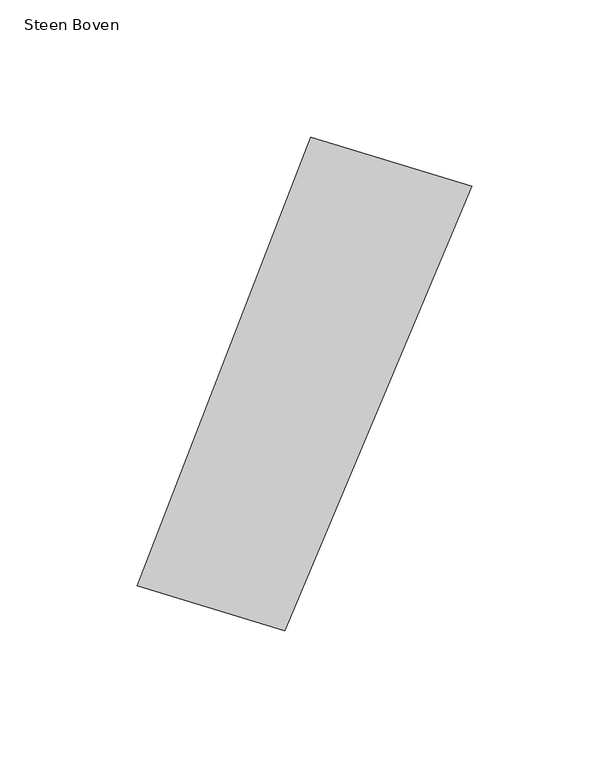
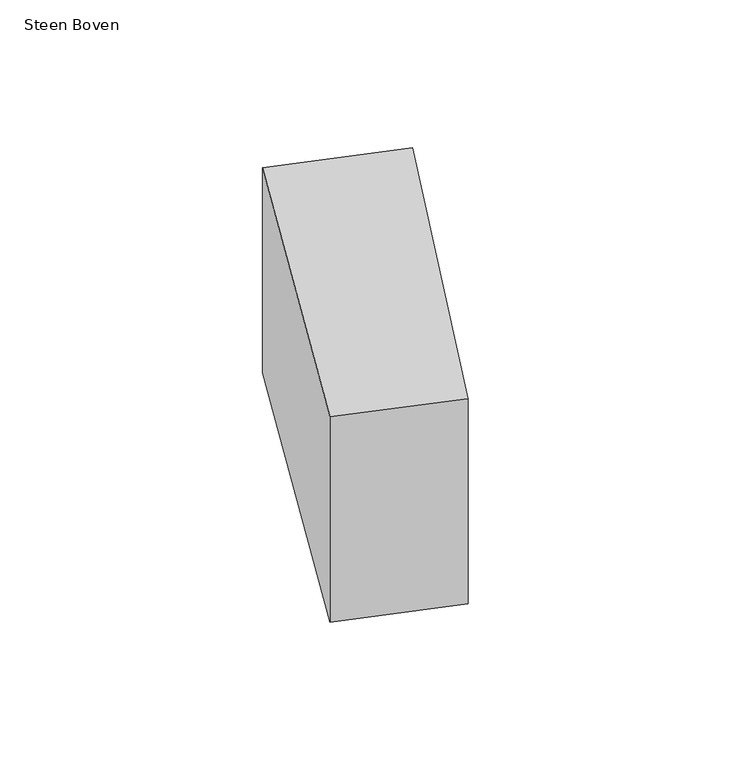
"""IFC4 building model written with IfcOpenShell, lengths in millimetres: proxy geometry, 00_GMA_steen_versie_4 : Steen Boven."""

from ifc_helpers import new_model, si_unit, origin, origin_with_axes, place, context, project, spatial, polyline, outline, extrude, source, transform, mapped, element, save


def steen_boven_2d31b367(model_context):
    return source(origin(), model_context, "Body", "SweptSolid", [
        extrude(outline(polyline([(135.7931837, 153.4581813), (67.6896866, -8.7195516), (13.7510423, 7.8523777), (77.070242, 171.4883092), (135.7931837, 153.4581813)])), origin_with_axes(), (0.0, 0.0, 1.0), 100.0),
    ])


if __name__ == "__main__":
    model = new_model("IFC4")
    model_context = context("Model", 3, world=origin())
    ifc_project = project(units=[si_unit("LENGTHUNIT", "METRE", prefix="MILLI")], contexts=[model_context])
    site = spatial("IfcSite", under=ifc_project)
    building = spatial("IfcBuilding", under=site)
    placement = place(None, origin())
    steen_boven_shape = steen_boven_2d31b367(model_context)
    element("IfcBuildingElementProxy", 1, Name="00_GMA_steen_versie_4 : Steen Boven", ObjectType="00_GMA_steen_versie_4 : Steen Boven", at=placement, inside=building, context=model_context, shape_type="MappedRepresentation", body=[
        mapped(steen_boven_shape, transform((0.0, 0.0, 0.0), x_axis=(1.0, 0.0, 0.0), y_axis=(0.0, 1.0, 0.0), z_axis=(0.0, 0.0, 1.0))),
    ])
    save(model, "model.ifc")

# Revit data of these elements
# Type "00_GMA_steen_versie_4 : Steen Boven"
#   StootVoegHalfBoven [instance default] = 5 mm
#   StootVoegHalf [instance default] = 5 mm
#   StootVoegBreedteOnder = 10 mm
#   StootVoegBreedteBoven = 10 mm
#   Steendikte = 100 mm
#   LintVoegOnderHalf = 5 mm
#   LintVoegOnder = 10 mm
#   LintVoegBovenHalf = 0 mm
#   LintVoegBoven = 0 mm
#   materiaal = none
#   MateriaalVoeg = none
#   Default Elevation = 0
